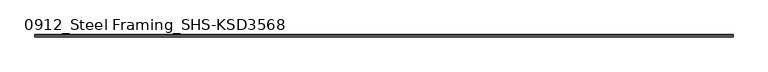
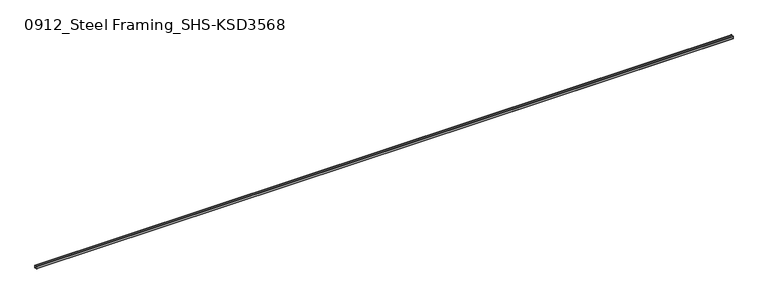
"""IFC4 building model written with IfcOpenShell, lengths in millimetres: beam geometry, 0912_Steel Framing_SHS-KSD3568 : H_SB_ASB_SHS-150x150x6."""

from ifc_helpers import new_model, si_unit, point, frame, frame_2d, origin, place, context, project, spatial, polyline, circle_curve, trimmed, segment, composite_curve, outline, extrude, source, transform, mapped, element, save


def beam_0912_steel_framing_shs_ksd3568_fce2b957(model_context):
    return source(origin(), model_context, "Body", "SweptSolid", [
        extrude(outline(composite_curve([segment(trimmed(circle_curve(frame_2d((-63.0, 63.0)), 12.0), [point((-75.0, 63.0))], [point((-63.0, 75.0))], False, "CARTESIAN"), True, "CONTINUOUS"), segment(polyline([(-63.0, 75.0), (63.0, 75.0)]), True, "CONTINUOUS"), segment(trimmed(circle_curve(frame_2d((63.0, 63.0)), 12.0), [point((63.0, 75.0))], [point((75.0, 63.0))], False, "CARTESIAN"), True, "CONTINUOUS"), segment(polyline([(75.0, 63.0), (75.0, -63.0)]), True, "CONTINUOUS"), segment(trimmed(circle_curve(frame_2d((63.0, -63.0)), 12.0), [point((75.0, -63.0))], [point((63.0, -75.0))], False, "CARTESIAN"), True, "CONTINUOUS"), segment(polyline([(63.0, -75.0), (-63.0, -75.0)]), True, "CONTINUOUS"), segment(trimmed(circle_curve(frame_2d((-63.0, -63.0)), 12.0), [point((-63.0, -75.0))], [point((-75.0, -63.0))], False, "CARTESIAN"), True, "CONTINUOUS"), segment(polyline([(-75.0, -63.0), (-75.0, 63.0)]), True, "CONTINUOUS")], self_intersect=False), holes=[composite_curve([segment(polyline([(63.0, 69.0), (-63.0, 69.0)]), True, "CONTINUOUS"), segment(trimmed(circle_curve(frame_2d((-63.0, 63.0)), 6.0), [point((-63.0, 69.0))], [point((-69.0, 63.0))], True, "CARTESIAN"), True, "CONTINUOUS"), segment(polyline([(-69.0, 63.0), (-69.0, -63.0)]), True, "CONTINUOUS"), segment(trimmed(circle_curve(frame_2d((-63.0, -63.0)), 6.0), [point((-69.0, -63.0))], [point((-63.0, -69.0))], True, "CARTESIAN"), True, "CONTINUOUS"), segment(polyline([(-63.0, -69.0), (63.0, -69.0)]), True, "CONTINUOUS"), segment(trimmed(circle_curve(frame_2d((63.0, -63.0)), 6.0), [point((63.0, -69.0))], [point((69.0, -63.0))], True, "CARTESIAN"), True, "CONTINUOUS"), segment(polyline([(69.0, -63.0), (69.0, 63.0)]), True, "CONTINUOUS"), segment(trimmed(circle_curve(frame_2d((63.0, 63.0)), 6.0), [point((69.0, 63.0))], [point((63.0, 69.0))], True, "CARTESIAN"), True, "CONTINUOUS")], self_intersect=False)]), frame((-20462.3, 0.0, 0.0), z_axis=(1.0, 0.0, 0.0), x_axis=(0.0, 1.0, 0.0)), (0.0, 0.0, 1.0), 40924.6),
    ])


if __name__ == "__main__":
    model = new_model("IFC4")
    model_context = context("Model", 3, world=origin())
    ifc_project = project(units=[si_unit("LENGTHUNIT", "METRE", prefix="MILLI")], contexts=[model_context])
    site = spatial("IfcSite", under=ifc_project)
    building = spatial("IfcBuilding", under=site)
    placement = place(None, origin())
    beam_0912_steel_framing_shs_ksd3568_shape = beam_0912_steel_framing_shs_ksd3568_fce2b957(model_context)
    element("IfcBeam", 1, ObjectType="0912_Steel Framing_SHS-KSD3568 : H_SB_ASB_SHS-150x150x6", at=placement, inside=building, context=model_context, shape_type="MappedRepresentation", body=[
        mapped(beam_0912_steel_framing_shs_ksd3568_shape, transform((0.0, 0.0, 0.0), x_axis=(1.0, 0.0, 0.0), y_axis=(0.0, 1.0, 0.0), z_axis=(0.0, 0.0, 1.0))),
    ])
    save(model, "model.ifc")

# Revit data of these elements
# Type "0912_Steel Framing_SHS-KSD3568 : H_SB_ASB_SHS-150x150x6"
#   H_WM Code_1 = "S01AA002-00001 | Main Steel Structure Fabrication Work | Shelter/Building | Medium Steel - Standard (90KG/M>Weight≥30KG/M) | Material: (   )"
#   H_WM Code_2 = "S03AA028-00001 | Main Steel Structure Erection Work | Shelter/Building | Medium Steel (90KG/M>Weight≥30KG/M) | Material: (   )"
#   H_WM Code_3 = "S01AA010-00001 | Main Steel Structure Fabrication Work | Shelter/Building | Steel Painting/Coating | for Non-Fireproofed Steel Surface, Surface Preparation, Primer, Second & Final Coat | Material: (   )"
#   H_Q'ty Cal Type Tag = "SB-Q2"
#   Perimeter = 0.60 m²/m
#   Nominal Weight = 26.40 kgf/m
#   Length [instance default] = 1.0000 m
#   b = 0.1500 m
#   h = 0.1500 m
#   tr = 0.0120 m
#   t = 0.0060 m
#   A = 28.36 m²
#   Structural Material [instance default] = Steel, 45-345
# Element 1 (IfcBeam, "0912_Steel Framing_SHS-KSD3568 : H_SB_ASB_SHS-150x150x6")
#   Structural Material = none
# Materials
#   "Steel, 45-345": class "Metal", colour RGB 189 187 185, transparency 0, Description = "Steel 345 MPa", Cost = 0
